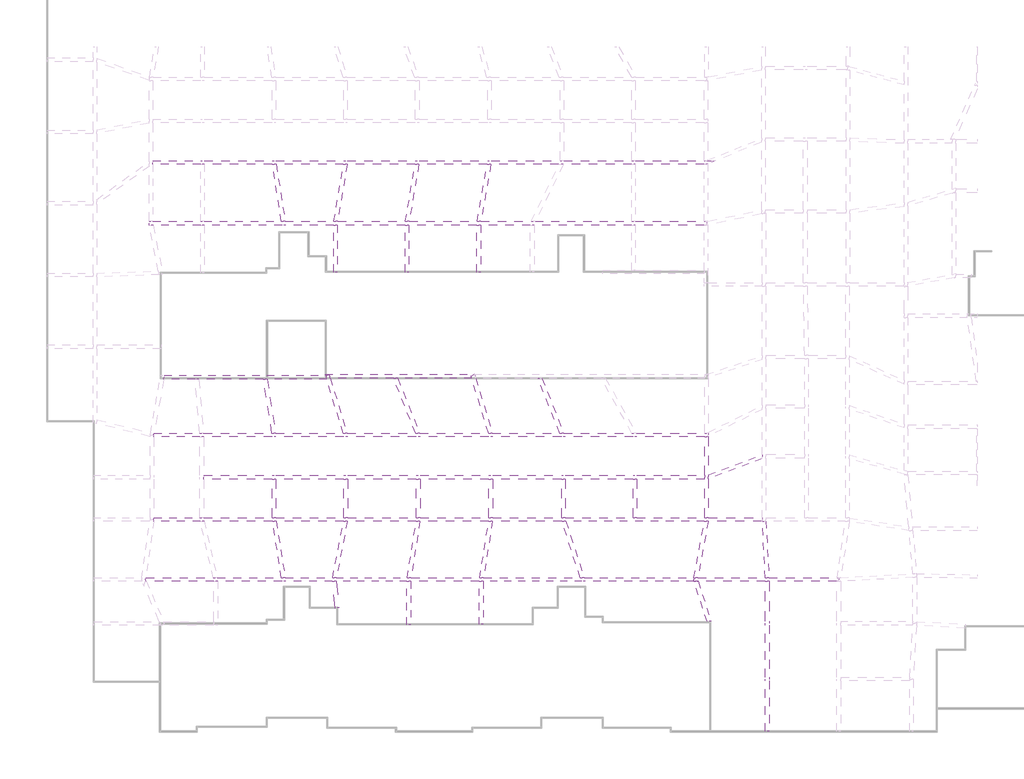
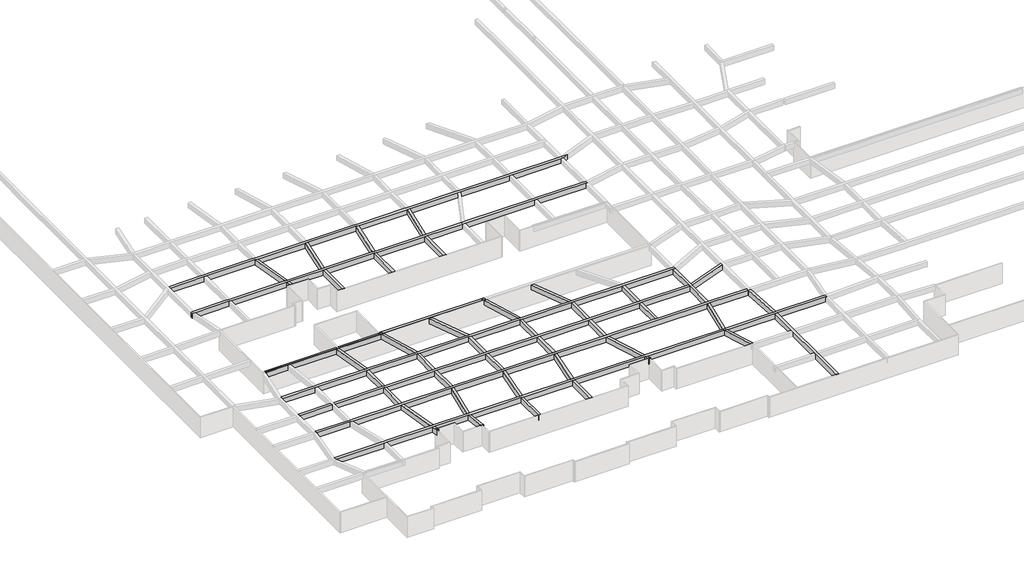
# One storey, part 11 of 45: 41 beams.
"""IFC4 building model written with IfcOpenShell, lengths in millimetres."""

from ifc_helpers import new_model, si_unit, frame, origin, place, context, project, spatial, polyline, outline, extrude, faceted_brep, element, save

model = new_model("IFC4")

# Units and contexts
model_context = context("Model", 3, world=origin())
ifc_project = project(units=[si_unit("LENGTHUNIT", "METRE", prefix="MILLI")], contexts=[model_context])

# Site, building, storey
site = spatial("IfcSite", under=ifc_project)
building = spatial("IfcBuilding", under=site)
storey = spatial("IfcBuildingStorey", under=building, Name="户型图", Elevation=0.0)

# Beams
placement = place(None, origin())
element("IfcBeam", 1, ObjectType="混凝土 - 矩形梁 : KL_beam", at=placement, inside=storey, context=model_context, shape_type="Brep", body=[
    faceted_brep([(-73789.7274974, -130269.3244435, 3300.0), (-73674.2267606, -130222.6591167, 3300.0), (-72799.6927561, -129869.3244435, 3300.0), (-73867.4796211, -129869.3244435, 3300.0), (-74074.2267606, -129869.3244435, 3300.0), (-81574.2267606, -129869.3244435, 3300.0), (-81974.2267606, -129869.3244435, 3300.0), (-89374.2267606, -129869.3244435, 3300.0), (-89774.2267606, -129869.3244435, 3300.0), (-97274.2267606, -129869.3244435, 3300.0), (-97674.2267606, -129869.3244435, 3300.0), (-105129.6078212, -129869.3244435, 3300.0), (-105529.6078212, -129869.3244435, 3300.0), (-112929.6078212, -129869.3244435, 3300.0), (-113329.6078212, -129869.3244435, 3300.0), (-120729.6078212, -129869.3244435, 3300.0), (-121129.6078212, -129869.3244435, 3300.0), (-128529.6078212, -129869.3244435, 3300.0), (-128929.6078212, -129869.3244435, 3300.0), (-134129.6078212, -129869.3244435, 3300.0), (-134129.6078212, -130269.3244435, 3300.0), (-128929.6078212, -130269.3244435, 3300.0), (-128529.6078212, -130269.3244435, 3300.0), (-121100.4239582, -130269.3244435, 3300.0), (-120695.4379079, -130269.3244435, 3300.0), (-113366.1859307, -130269.3244435, 3300.0), (-112960.5304704, -130269.3244435, 3300.0), (-105566.1859307, -130269.3244435, 3300.0), (-105160.5304704, -130269.3244435, 3300.0), (-97712.5774791, -130269.3244435, 3300.0), (-97306.4068344, -130269.3244435, 3300.0), (-89894.2936664, -130269.3244435, 3300.0), (-89449.2528902, -130269.3244435, 3300.0), (-81974.2267606, -130269.3244435, 3300.0), (-81574.2267606, -130269.3244435, 3300.0), (-74074.2267606, -130269.3244435, 3300.0), (-73789.7274974, -130269.3244435, 2500.0), (-134129.6078212, -130269.3244435, 2500.0), (-128929.6078212, -130269.3244435, 2500.0), (-128529.6078212, -130269.3244435, 2500.0), (-121100.4239582, -130269.3244435, 2500.0), (-120695.4379079, -130269.3244435, 2500.0), (-113366.1859307, -130269.3244435, 2500.0), (-112960.5304704, -130269.3244435, 2500.0), (-105566.1859307, -130269.3244435, 2500.0), (-105160.5304704, -130269.3244435, 2500.0), (-97712.5774791, -130269.3244435, 2500.0), (-97306.4068344, -130269.3244435, 2500.0), (-89894.2936664, -130269.3244435, 2500.0), (-89449.2528902, -130269.3244435, 2500.0), (-81974.2267606, -130269.3244435, 2500.0), (-81574.2267606, -130269.3244435, 2500.0), (-74074.2267606, -130269.3244435, 2500.0), (-72799.6927561, -129869.3244435, 2500.0), (-73674.2267606, -130222.6591167, 2500.0), (-134129.6078212, -129869.3244435, 2500.0), (-128929.6078212, -129869.3244435, 2500.0), (-128529.6078212, -129869.3244435, 2500.0), (-121129.6078212, -129869.3244435, 2500.0), (-120729.6078212, -129869.3244435, 2500.0), (-113329.6078212, -129869.3244435, 2500.0), (-112929.6078212, -129869.3244435, 2500.0), (-105529.6078212, -129869.3244435, 2500.0), (-105129.6078212, -129869.3244435, 2500.0), (-97674.2267606, -129869.3244435, 2500.0), (-97274.2267606, -129869.3244435, 2500.0), (-89774.2267606, -129869.3244435, 2500.0), (-89374.2267606, -129869.3244435, 2500.0), (-81974.2267606, -129869.3244435, 2500.0), (-81574.2267606, -129869.3244435, 2500.0), (-74074.2267606, -129869.3244435, 2500.0), (-73867.4796211, -129869.3244435, 2500.0)], [[[0, 1, 2, 3, 4, 5, 6, 7, 8, 9, 10, 11, 12, 13, 14, 15, 16, 17, 18, 19, 20, 21, 22, 23, 24, 25, 26, 27, 28, 29, 30, 31, 32, 33, 34, 35]], [[36, 0, 35, 34, 33, 32, 31, 30, 29, 28, 27, 26, 25, 24, 23, 22, 21, 20, 37, 38, 39, 40, 41, 42, 43, 44, 45, 46, 47, 48, 49, 50, 51, 52]], [[53, 54, 36, 52, 51, 50, 49, 48, 47, 46, 45, 44, 43, 42, 41, 40, 39, 38, 37, 55, 56, 57, 58, 59, 60, 61, 62, 63, 64, 65, 66, 67, 68, 69, 70, 71]], [[2, 53, 71, 70, 69, 68, 67, 66, 65, 64, 63, 62, 61, 60, 59, 58, 57, 56, 55, 19, 18, 17, 16, 15, 14, 13, 12, 11, 10, 9, 8, 7, 6, 5, 4, 3]], [[20, 19, 55, 37]], [[2, 1, 0, 36, 54, 53]]]),
])
element("IfcBeam", 2, ObjectType="混凝土 - 矩形梁 : KL_beam", at=placement, inside=storey, context=model_context, shape_type="Brep", body=[
    faceted_brep([(-73801.0394369, -136882.7394466, 3300.0), (-73841.6921627, -136482.7394466, 3300.0), (-74074.2267606, -136482.7394466, 3300.0), (-81574.2267606, -136482.7394466, 3300.0), (-81974.2267606, -136482.7394466, 3300.0), (-92479.7378735, -136482.7394466, 3300.0), (-92924.7786497, -136482.7394466, 3300.0), (-98401.9995417, -136482.7394466, 3300.0), (-98808.1701865, -136482.7394466, 3300.0), (-106209.0560389, -136482.7394466, 3300.0), (-106614.7114991, -136482.7394466, 3300.0), (-114009.0560389, -136482.7394466, 3300.0), (-114414.7114991, -136482.7394466, 3300.0), (-119711.3296502, -136482.7394466, 3300.0), (-120116.3157005, -136482.7394466, 3300.0), (-128529.6078212, -136482.7394466, 3300.0), (-128929.6078212, -136482.7394466, 3300.0), (-134129.6078212, -136482.7394466, 3300.0), (-134529.6078212, -136482.7394466, 3300.0), (-134529.6078212, -136882.7394466, 3300.0), (-134494.0876303, -136882.7394466, 3300.0), (-134086.4357741, -136882.7394466, 3300.0), (-128929.6078212, -136882.7394466, 3300.0), (-128529.6078212, -136882.7394466, 3300.0), (-120052.9619243, -136882.7394466, 3300.0), (-119647.975874, -136882.7394466, 3300.0), (-114445.6408237, -136882.7394466, 3300.0), (-114045.6408237, -136882.7394466, 3300.0), (-106645.6408237, -136882.7394466, 3300.0), (-106245.6408237, -136882.7394466, 3300.0), (-98840.399091, -136882.7394466, 3300.0), (-98440.399091, -136882.7394466, 3300.0), (-93000.0024046, -136882.7394466, 3300.0), (-92600.0024046, -136882.7394466, 3300.0), (-81974.2267606, -136882.7394466, 3300.0), (-81574.2267606, -136882.7394466, 3300.0), (-74074.2267606, -136882.7394466, 3300.0), (-73801.0394369, -136882.7394466, 2500.0), (-134529.6078212, -136882.7394466, 2500.0), (-134494.0876303, -136882.7394466, 2500.0), (-134086.4357741, -136882.7394466, 2500.0), (-128929.6078212, -136882.7394466, 2500.0), (-128529.6078212, -136882.7394466, 2500.0), (-120052.9619243, -136882.7394466, 2500.0), (-119647.975874, -136882.7394466, 2500.0), (-114445.6408237, -136882.7394466, 2500.0), (-114045.6408237, -136882.7394466, 2500.0), (-106645.6408237, -136882.7394466, 2500.0), (-106245.6408237, -136882.7394466, 2500.0), (-98840.399091, -136882.7394466, 2500.0), (-98440.399091, -136882.7394466, 2500.0), (-93000.0024046, -136882.7394466, 2500.0), (-92600.0024046, -136882.7394466, 2500.0), (-81974.2267606, -136882.7394466, 2500.0), (-81574.2267606, -136882.7394466, 2500.0), (-74074.2267606, -136882.7394466, 2500.0), (-73841.6921627, -136482.7394466, 2500.0), (-134529.6078212, -136482.7394466, 2500.0), (-134129.6078212, -136482.7394466, 2500.0), (-128929.6078212, -136482.7394466, 2500.0), (-128529.6078212, -136482.7394466, 2500.0), (-120116.3157005, -136482.7394466, 2500.0), (-119711.3296502, -136482.7394466, 2500.0), (-114414.7114991, -136482.7394466, 2500.0), (-114009.0560389, -136482.7394466, 2500.0), (-106614.7114991, -136482.7394466, 2500.0), (-106209.0560389, -136482.7394466, 2500.0), (-98808.1701865, -136482.7394466, 2500.0), (-98401.9995417, -136482.7394466, 2500.0), (-92924.7786497, -136482.7394466, 2500.0), (-92479.7378735, -136482.7394466, 2500.0), (-81974.2267606, -136482.7394466, 2500.0), (-81574.2267606, -136482.7394466, 2500.0), (-74074.2267606, -136482.7394466, 2500.0)], [[[0, 1, 2, 3, 4, 5, 6, 7, 8, 9, 10, 11, 12, 13, 14, 15, 16, 17, 18, 19, 20, 21, 22, 23, 24, 25, 26, 27, 28, 29, 30, 31, 32, 33, 34, 35, 36]], [[37, 0, 36, 35, 34, 33, 32, 31, 30, 29, 28, 27, 26, 25, 24, 23, 22, 21, 20, 19, 38, 39, 40, 41, 42, 43, 44, 45, 46, 47, 48, 49, 50, 51, 52, 53, 54, 55]], [[56, 37, 55, 54, 53, 52, 51, 50, 49, 48, 47, 46, 45, 44, 43, 42, 41, 40, 39, 38, 57, 58, 59, 60, 61, 62, 63, 64, 65, 66, 67, 68, 69, 70, 71, 72, 73]], [[1, 56, 73, 72, 71, 70, 69, 68, 67, 66, 65, 64, 63, 62, 61, 60, 59, 58, 57, 18, 17, 16, 15, 14, 13, 12, 11, 10, 9, 8, 7, 6, 5, 4, 3, 2]], [[19, 18, 57, 38]], [[1, 0, 37, 56]]]),
])
element("IfcBeam", 3, ObjectType="混凝土 - 矩形梁 : KL_beam", at=placement, inside=storey, context=model_context, shape_type="SweptSolid", body=[
    extrude(outline(polyline([(-105566.1859307, -130269.3244435), (-105160.5304704, -130269.3244435), (-106209.0560389, -136482.7394466), (-106614.7114991, -136482.7394466), (-105566.1859307, -130269.3244435)])), frame((0.0, 0.0, 2500.0), z_axis=(0.0, 0.0, 1.0), x_axis=(1.0, 0.0, 0.0)), (0.0, 0.0, 1.0), 800.0),
])
element("IfcBeam", 4, ObjectType="混凝土 - 矩形梁 : KL_beam", at=placement, inside=storey, context=model_context, shape_type="SweptSolid", body=[
    extrude(outline(polyline([(-113366.1859307, -130269.3244435), (-112960.5304704, -130269.3244435), (-114009.0560389, -136482.7394466), (-114414.7114991, -136482.7394466), (-113366.1859307, -130269.3244435)])), frame((0.0, 0.0, 2500.0), z_axis=(0.0, 0.0, 1.0), x_axis=(1.0, 0.0, 0.0)), (0.0, 0.0, 1.0), 800.0),
])
element("IfcBeam", 5, ObjectType="混凝土 - 矩形梁 : KL_beam", at=placement, inside=storey, context=model_context, shape_type="SweptSolid", body=[
    extrude(outline(polyline([(-97712.5774791, -130269.3244435), (-97306.4068344, -130269.3244435), (-98401.9995417, -136482.7394466), (-98808.1701865, -136482.7394466), (-97712.5774791, -130269.3244435)])), frame((0.0, 0.0, 2500.0), z_axis=(0.0, 0.0, 1.0), x_axis=(1.0, 0.0, 0.0)), (0.0, 0.0, 1.0), 800.0),
])
element("IfcBeam", 6, ObjectType="混凝土 - 矩形梁 : KL_beam", at=placement, inside=storey, context=model_context, shape_type="SweptSolid", body=[
    extrude(outline(polyline([(-98440.399091, -141990.9010637), (-98840.399091, -141990.9010637), (-98840.399091, -136882.7394466), (-98440.399091, -136882.7394466), (-98440.399091, -141990.9010637)])), frame((0.0, 0.0, 2500.0), z_axis=(0.0, 0.0, 1.0), x_axis=(1.0, 0.0, 0.0)), (0.0, 0.0, 1.0), 800.0),
])
element("IfcBeam", 7, ObjectType="混凝土 - 矩形梁 : KL_beam", at=placement, inside=storey, context=model_context, shape_type="Brep", body=[
    faceted_brep([(-75195.4874183, -175680.7215365, 3300.0), (-74862.8225004, -175680.7215365, 3300.0), (-74755.4433093, -175680.7215365, 3300.0), (-67421.4283331, -175680.7215365, 3300.0), (-67021.4283331, -175680.7215365, 3300.0), (-59629.7273676, -175680.7215365, 3300.0), (-59424.4901833, -175680.7215365, 3300.0), (-59434.9645519, -175280.7215365, 3300.0), (-59602.3197398, -175280.7215365, 3300.0), (-67031.6354197, -175280.7215365, 3300.0), (-67432.1843581, -175280.7215365, 3300.0), (-74788.6727332, -175280.7215365, 3300.0), (-75195.4874183, -175280.7215365, 3300.0), (-75195.4874183, -175283.8093857, 3300.0), (-59434.9645519, -175280.7215365, 2500.0), (-59602.3197398, -175280.7215365, 2500.0), (-67031.6354197, -175280.7215365, 2500.0), (-67432.1843581, -175280.7215365, 2500.0), (-74788.6727332, -175280.7215365, 2500.0), (-75195.4874183, -175280.7215365, 2500.0), (-59424.4901833, -175680.7215365, 2500.0), (-59629.7273676, -175680.7215365, 2500.0), (-67021.4283331, -175680.7215365, 2500.0), (-67421.4283331, -175680.7215365, 2500.0), (-74755.4433093, -175680.7215365, 2500.0), (-74862.8225004, -175680.7215365, 2500.0), (-75195.4874183, -175680.7215365, 2500.0), (-75195.4874183, -175283.8093857, 2500.0)], [[[0, 1, 2, 3, 4, 5, 6, 7, 8, 9, 10, 11, 12, 13]], [[12, 11, 10, 9, 8, 7, 14, 15, 16, 17, 18, 19]], [[19, 18, 17, 16, 15, 14, 20, 21, 22, 23, 24, 25, 26, 27]], [[6, 5, 4, 3, 2, 1, 0, 26, 25, 24, 23, 22, 21, 20]], [[6, 20, 14, 7]], [[0, 13, 12, 19, 27, 26]]]),
])
element("IfcBeam", 8, ObjectType="混凝土 - 矩形梁 : KL_beam", at=placement, inside=storey, context=model_context, shape_type="Brep", body=[
    faceted_brep([(-67352.9383994, -169149.8954633, 3300.0), (-67363.6944245, -169149.8954633, 3300.0), (-67753.4873378, -169149.8954633, 3300.0), (-67432.1843581, -175280.7215365, 3300.0), (-67031.6354197, -175280.7215365, 3300.0), (-67753.4873378, -169149.8954633, 2500.0), (-67432.1843581, -175280.7215365, 2500.0), (-67363.6944245, -169149.8954633, 2500.0), (-67352.9383994, -169149.8954633, 2500.0), (-67031.6354197, -175280.7215365, 2500.0)], [[[0, 1, 2, 3, 4]], [[2, 5, 6, 3]], [[5, 7, 8, 9, 6]], [[8, 0, 4, 9]], [[5, 2, 1, 0, 8, 7]], [[4, 3, 6, 9]]]),
    faceted_brep([(-67763.6944245, -168955.1326476, 3300.0), (-67763.6944245, -168955.1326476, 2500.0), (-67763.6944245, -168749.8954633, 2500.0), (-67763.6944245, -168748.040132, 2500.0), (-67763.6944245, -168748.040132, 3300.0), (-67763.6944245, -168749.8954633, 3300.0), (-67774.5476833, -168748.040132, 2500.0), (-67774.5476833, -168748.040132, 3300.0)], [[[0, 1, 2, 3, 4, 5]], [[6, 7, 4, 3]], [[7, 0, 5, 4]], [[0, 7, 6, 1]], [[1, 6, 3, 2]]]),
])
element("IfcBeam", 9, ObjectType="混凝土 - 矩形梁 : KL_beam", at=placement, inside=storey, context=model_context, shape_type="Brep", body=[
    faceted_brep([(-67021.4283331, -192027.8669315, 3300.0), (-67421.4283331, -192027.8669315, 3300.0), (-67421.4283331, -192027.8669315, 2500.0), (-67021.4283331, -192027.8669315, 2500.0), (-67021.4283331, -186528.0123265, 3300.0), (-67021.4283331, -186128.0123265, 3300.0), (-67021.4283331, -180443.730522, 3300.0), (-67021.4283331, -180043.730522, 3300.0), (-67021.4283331, -175680.7215365, 3300.0), (-67421.4283331, -175680.7215365, 3300.0), (-67421.4283331, -180043.730522, 3300.0), (-67421.4283331, -180443.730522, 3300.0), (-67421.4283331, -186128.0123265, 3300.0), (-67421.4283331, -186528.0123265, 3300.0), (-67421.4283331, -175680.7215365, 2500.0), (-67421.4283331, -180043.730522, 2500.0), (-67421.4283331, -180443.730522, 2500.0), (-67421.4283331, -186128.0123265, 2500.0), (-67421.4283331, -186528.0123265, 2500.0), (-67021.4283331, -175680.7215365, 2500.0), (-67021.4283331, -180043.730522, 2500.0), (-67021.4283331, -180443.730522, 2500.0), (-67021.4283331, -186128.0123265, 2500.0), (-67021.4283331, -186528.0123265, 2500.0)], [[[0, 1, 2, 3]], [[1, 0, 4, 5, 6, 7, 8, 9, 10, 11, 12, 13]], [[2, 1, 13, 12, 11, 10, 9, 14, 15, 16, 17, 18]], [[3, 2, 18, 17, 16, 15, 14, 19, 20, 21, 22, 23]], [[0, 3, 23, 22, 21, 20, 19, 8, 7, 6, 5, 4]], [[9, 8, 19, 14]]]),
])
element("IfcBeam", 10, ObjectType="混凝土 - 矩形梁 : KL_beam", at=placement, inside=storey, context=model_context, shape_type="SweptSolid", body=[
    extrude(outline(polyline([(-119527.5247722, -137643.237773), (-119922.6001085, -137705.8115591), (-120052.9619243, -136882.7394466), (-119647.975874, -136882.7394466), (-119527.5247722, -137643.237773)])), frame((0.0, 0.0, 2500.0), z_axis=(0.0, 0.0, 1.0), x_axis=(1.0, 0.0, 0.0)), (0.0, 0.0, 1.0), 800.0),
    extrude(outline(polyline([(-121100.4239582, -130269.3244435), (-120695.4379079, -130269.3244435), (-119711.3296502, -136482.7394466), (-120116.3157005, -136482.7394466), (-121100.4239582, -130269.3244435)])), frame((0.0, 0.0, 2500.0), z_axis=(0.0, 0.0, 1.0), x_axis=(1.0, 0.0, 0.0)), (0.0, 0.0, 1.0), 800.0),
])
element("IfcBeam", 11, ObjectType="混凝土 - 矩形梁 : KL_beam", at=placement, inside=storey, context=model_context, shape_type="Brep", body=[
    faceted_brep([(-134906.6317316, -175283.8093857, 3300.0), (-134930.932576, -175456.7188778, 3300.0), (-134834.5383744, -175683.8093857, 3300.0), (-127468.1198938, -175683.8093857, 3300.0), (-127068.1198938, -175683.8093857, 3300.0), (-120053.8149285, -175683.8093857, 3300.0), (-119648.8288782, -175683.8093857, 3300.0), (-114567.3022088, -175683.8093857, 3300.0), (-114164.7670122, -175683.8093857, 3300.0), (-106453.3866692, -175683.8093857, 3300.0), (-106053.3866692, -175683.8093857, 3300.0), (-98553.3271021, -175683.8093857, 3300.0), (-98153.3271021, -175683.8093857, 3300.0), (-87439.8712918, -175683.8093857, 3300.0), (-87019.2864021, -175683.8093857, 3300.0), (-75175.0248959, -175683.8093857, 3300.0), (-74863.3949086, -175683.8093857, 3300.0), (-74862.8225004, -175680.7215365, 3300.0), (-75195.4874183, -175680.7215365, 3300.0), (-75195.4874183, -175283.8093857, 3300.0), (-87149.2542806, -175283.8093857, 3300.0), (-87569.8391703, -175283.8093857, 3300.0), (-98119.1571889, -175283.8093857, 3300.0), (-98524.1432392, -175283.8093857, 3300.0), (-106019.1571889, -175283.8093857, 3300.0), (-106424.1432392, -175283.8093857, 3300.0), (-114145.9683939, -175283.8093857, 3300.0), (-114553.4550719, -175283.8093857, 3300.0), (-119712.1826543, -175283.8093857, 3300.0), (-120117.1687046, -175283.8093857, 3300.0), (-127122.7494049, -175283.8093857, 3300.0), (-127533.271048, -175283.8093857, 3300.0), (-134834.5383744, -175683.8093857, 2500.0), (-127468.1198938, -175683.8093857, 2500.0), (-127068.1198938, -175683.8093857, 2500.0), (-120053.8149285, -175683.8093857, 2500.0), (-119648.8288782, -175683.8093857, 2500.0), (-114567.3022088, -175683.8093857, 2500.0), (-114164.7670122, -175683.8093857, 2500.0), (-106453.3866692, -175683.8093857, 2500.0), (-106053.3866692, -175683.8093857, 2500.0), (-98553.3271021, -175683.8093857, 2500.0), (-98153.3271021, -175683.8093857, 2500.0), (-87439.8712918, -175683.8093857, 2500.0), (-87019.2864021, -175683.8093857, 2500.0), (-75175.0248959, -175683.8093857, 2500.0), (-74863.3949086, -175683.8093857, 2500.0), (-134930.932576, -175456.7188778, 2500.0), (-134906.6317316, -175283.8093857, 2500.0), (-127533.271048, -175283.8093857, 2500.0), (-127122.7494049, -175283.8093857, 2500.0), (-120117.1687046, -175283.8093857, 2500.0), (-119712.1826543, -175283.8093857, 2500.0), (-114553.4550719, -175283.8093857, 2500.0), (-114145.9683939, -175283.8093857, 2500.0), (-106424.1432392, -175283.8093857, 2500.0), (-106019.1571889, -175283.8093857, 2500.0), (-98524.1432392, -175283.8093857, 2500.0), (-98119.1571889, -175283.8093857, 2500.0), (-87569.8391703, -175283.8093857, 2500.0), (-87149.2542806, -175283.8093857, 2500.0), (-75195.4874183, -175283.8093857, 2500.0), (-75195.4874183, -175680.7215365, 2500.0), (-74862.8225004, -175680.7215365, 2500.0)], [[[0, 1, 2, 3, 4, 5, 6, 7, 8, 9, 10, 11, 12, 13, 14, 15, 16, 17, 18, 19, 20, 21, 22, 23, 24, 25, 26, 27, 28, 29, 30, 31]], [[2, 32, 33, 34, 35, 36, 37, 38, 39, 40, 41, 42, 43, 44, 45, 46, 16, 15, 14, 13, 12, 11, 10, 9, 8, 7, 6, 5, 4, 3]], [[47, 48, 49, 50, 51, 52, 53, 54, 55, 56, 57, 58, 59, 60, 61, 62, 63, 46, 45, 44, 43, 42, 41, 40, 39, 38, 37, 36, 35, 34, 33, 32]], [[48, 0, 31, 30, 29, 28, 27, 26, 25, 24, 23, 22, 21, 20, 19, 61, 60, 59, 58, 57, 56, 55, 54, 53, 52, 51, 50, 49]], [[0, 48, 47, 1]], [[2, 1, 47, 32]], [[62, 18, 17, 63]], [[18, 62, 61, 19]], [[16, 46, 63, 17]]]),
])
element("IfcBeam", 12, ObjectType="混凝土 - 矩形梁 : KL_beam", at=placement, inside=storey, context=model_context, shape_type="Brep", body=[
    faceted_brep([(-67763.6944245, -169148.040132, 3300.0), (-67763.6944245, -168955.1326476, 3300.0), (-67774.5476833, -168748.040132, 3300.0), (-73618.1629467, -168748.040132, 3300.0), (-74018.1629467, -168748.040132, 3300.0), (-81418.1629467, -168748.040132, 3300.0), (-81818.1629467, -168748.040132, 3300.0), (-89218.1629467, -168748.040132, 3300.0), (-89618.1629467, -168748.040132, 3300.0), (-97118.1629467, -168748.040132, 3300.0), (-97518.1629467, -168748.040132, 3300.0), (-105018.1629467, -168748.040132, 3300.0), (-105418.1629467, -168748.040132, 3300.0), (-112918.1629467, -168748.040132, 3300.0), (-113318.1629467, -168748.040132, 3300.0), (-120718.1629467, -168748.040132, 3300.0), (-121118.1629467, -168748.040132, 3300.0), (-128597.7870634, -168748.040132, 3300.0), (-128997.7870634, -168748.040132, 3300.0), (-134018.1629467, -168748.040132, 3300.0), (-134018.1629467, -168962.0254944, 3300.0), (-134044.3055992, -169148.040132, 3300.0), (-128949.8249968, -169148.040132, 3300.0), (-128539.3033537, -169148.040132, 3300.0), (-121088.9790838, -169148.040132, 3300.0), (-120683.9930335, -169148.040132, 3300.0), (-113360.7823476, -169148.040132, 3300.0), (-112953.2956696, -169148.040132, 3300.0), (-105452.33286, -169148.040132, 3300.0), (-105047.3468096, -169148.040132, 3300.0), (-97552.33286, -169148.040132, 3300.0), (-97147.3468096, -169148.040132, 3300.0), (-89563.4714523, -169148.040132, 3300.0), (-89142.8865626, -169148.040132, 3300.0), (-74058.6451728, -169148.040132, 3300.0), (-73651.8304878, -169148.040132, 3300.0), (-67763.6944245, -169148.040132, 2500.0), (-134044.3055992, -169148.040132, 2500.0), (-128949.8249968, -169148.040132, 2500.0), (-128539.3033537, -169148.040132, 2500.0), (-121088.9790838, -169148.040132, 2500.0), (-120683.9930335, -169148.040132, 2500.0), (-113360.7823476, -169148.040132, 2500.0), (-112953.2956696, -169148.040132, 2500.0), (-105452.33286, -169148.040132, 2500.0), (-105047.3468096, -169148.040132, 2500.0), (-97552.33286, -169148.040132, 2500.0), (-97147.3468096, -169148.040132, 2500.0), (-89563.4714523, -169148.040132, 2500.0), (-89142.8865626, -169148.040132, 2500.0), (-74058.6451728, -169148.040132, 2500.0), (-73651.8304878, -169148.040132, 2500.0), (-67763.6944245, -168955.1326476, 2500.0), (-134018.1629467, -168962.0254944, 2500.0), (-134018.1629467, -168748.040132, 2500.0), (-128997.7870634, -168748.040132, 2500.0), (-128597.7870634, -168748.040132, 2500.0), (-121118.1629467, -168748.040132, 2500.0), (-120718.1629467, -168748.040132, 2500.0), (-113318.1629467, -168748.040132, 2500.0), (-112918.1629467, -168748.040132, 2500.0), (-105418.1629467, -168748.040132, 2500.0), (-105018.1629467, -168748.040132, 2500.0), (-97518.1629467, -168748.040132, 2500.0), (-97118.1629467, -168748.040132, 2500.0), (-89618.1629467, -168748.040132, 2500.0), (-89218.1629467, -168748.040132, 2500.0), (-81818.1629467, -168748.040132, 2500.0), (-81418.1629467, -168748.040132, 2500.0), (-74018.1629467, -168748.040132, 2500.0), (-73618.1629467, -168748.040132, 2500.0), (-67774.5476833, -168748.040132, 2500.0)], [[[0, 1, 2, 3, 4, 5, 6, 7, 8, 9, 10, 11, 12, 13, 14, 15, 16, 17, 18, 19, 20, 21, 22, 23, 24, 25, 26, 27, 28, 29, 30, 31, 32, 33, 34, 35]], [[36, 0, 35, 34, 33, 32, 31, 30, 29, 28, 27, 26, 25, 24, 23, 22, 21, 37, 38, 39, 40, 41, 42, 43, 44, 45, 46, 47, 48, 49, 50, 51]], [[52, 36, 51, 50, 49, 48, 47, 46, 45, 44, 43, 42, 41, 40, 39, 38, 37, 53, 54, 55, 56, 57, 58, 59, 60, 61, 62, 63, 64, 65, 66, 67, 68, 69, 70, 71]], [[2, 71, 70, 69, 68, 67, 66, 65, 64, 63, 62, 61, 60, 59, 58, 57, 56, 55, 54, 19, 18, 17, 16, 15, 14, 13, 12, 11, 10, 9, 8, 7, 6, 5, 4, 3]], [[0, 36, 52, 1]], [[2, 1, 52, 71]], [[20, 19, 54, 53]], [[21, 20, 53, 37]]]),
])
element("IfcBeam", 13, ObjectType="混凝土 - 矩形梁 : KL_beam", at=placement, inside=storey, context=model_context, shape_type="Brep", body=[
    faceted_brep([(-134018.1629467, -164148.040132, 3300.0), (-134018.1629467, -164548.040132, 3300.0), (-128997.7870634, -164548.040132, 3300.0), (-128997.7870634, -164148.040132, 3300.0), (-134018.1629467, -164548.040132, 2500.0), (-128997.7870634, -164548.040132, 2500.0), (-134018.1629467, -164148.040132, 2500.0), (-128997.7870634, -164148.040132, 2500.0)], [[[0, 1, 2, 3]], [[1, 4, 5, 2]], [[4, 6, 7, 5]], [[6, 0, 3, 7]], [[1, 0, 6, 4]], [[3, 2, 5, 7]]]),
    faceted_brep([(-128597.7870634, -164548.040132, 3300.0), (-128597.7870634, -164148.040132, 3300.0), (-128597.7870634, -164148.040132, 2500.0), (-128597.7870634, -164548.040132, 2500.0), (-121118.1629467, -164548.040132, 3300.0), (-120718.1629467, -164548.040132, 3300.0), (-113318.1629467, -164548.040132, 3300.0), (-112918.1629467, -164548.040132, 3300.0), (-105418.1629467, -164548.040132, 3300.0), (-105018.1629467, -164548.040132, 3300.0), (-97518.1629467, -164548.040132, 3300.0), (-97118.1629467, -164548.040132, 3300.0), (-89618.1629467, -164548.040132, 3300.0), (-89218.1629467, -164548.040132, 3300.0), (-81818.1629467, -164548.040132, 3300.0), (-81418.1629467, -164548.040132, 3300.0), (-74018.1629467, -164548.040132, 3300.0), (-74018.1629467, -164148.040132, 3300.0), (-81418.1629467, -164148.040132, 3300.0), (-81818.1629467, -164148.040132, 3300.0), (-89218.1629467, -164148.040132, 3300.0), (-89618.1629467, -164148.040132, 3300.0), (-97118.1629467, -164148.040132, 3300.0), (-97518.1629467, -164148.040132, 3300.0), (-105018.1629467, -164148.040132, 3300.0), (-105418.1629467, -164148.040132, 3300.0), (-112918.1629467, -164148.040132, 3300.0), (-113318.1629467, -164148.040132, 3300.0), (-120718.1629467, -164148.040132, 3300.0), (-121118.1629467, -164148.040132, 3300.0), (-121118.1629467, -164548.040132, 2500.0), (-120718.1629467, -164548.040132, 2500.0), (-113318.1629467, -164548.040132, 2500.0), (-112918.1629467, -164548.040132, 2500.0), (-105418.1629467, -164548.040132, 2500.0), (-105018.1629467, -164548.040132, 2500.0), (-97518.1629467, -164548.040132, 2500.0), (-97118.1629467, -164548.040132, 2500.0), (-89618.1629467, -164548.040132, 2500.0), (-89218.1629467, -164548.040132, 2500.0), (-81818.1629467, -164548.040132, 2500.0), (-81418.1629467, -164548.040132, 2500.0), (-74018.1629467, -164548.040132, 2500.0), (-121118.1629467, -164148.040132, 2500.0), (-120718.1629467, -164148.040132, 2500.0), (-113318.1629467, -164148.040132, 2500.0), (-112918.1629467, -164148.040132, 2500.0), (-105418.1629467, -164148.040132, 2500.0), (-105018.1629467, -164148.040132, 2500.0), (-97518.1629467, -164148.040132, 2500.0), (-97118.1629467, -164148.040132, 2500.0), (-89618.1629467, -164148.040132, 2500.0), (-89218.1629467, -164148.040132, 2500.0), (-81818.1629467, -164148.040132, 2500.0), (-81418.1629467, -164148.040132, 2500.0), (-74018.1629467, -164148.040132, 2500.0)], [[[0, 1, 2, 3]], [[1, 0, 4, 5, 6, 7, 8, 9, 10, 11, 12, 13, 14, 15, 16, 17, 18, 19, 20, 21, 22, 23, 24, 25, 26, 27, 28, 29]], [[0, 3, 30, 31, 32, 33, 34, 35, 36, 37, 38, 39, 40, 41, 42, 16, 15, 14, 13, 12, 11, 10, 9, 8, 7, 6, 5, 4]], [[3, 2, 43, 44, 45, 46, 47, 48, 49, 50, 51, 52, 53, 54, 55, 42, 41, 40, 39, 38, 37, 36, 35, 34, 33, 32, 31, 30]], [[2, 1, 29, 28, 27, 26, 25, 24, 23, 22, 21, 20, 19, 18, 17, 55, 54, 53, 52, 51, 50, 49, 48, 47, 46, 45, 44, 43]], [[17, 16, 42, 55]]]),
])
element("IfcBeam", 14, ObjectType="混凝土 - 矩形梁 : KL_beam", at=placement, inside=storey, context=model_context, shape_type="Brep", body=[
    faceted_brep([(-134018.1629467, -159765.5378647, 3300.0), (-134018.1629467, -159948.040132, 3300.0), (-128997.7870634, -159948.040132, 3300.0), (-128597.7870634, -159948.040132, 3300.0), (-121118.1629467, -159948.040132, 3300.0), (-120718.1629467, -159948.040132, 3300.0), (-113318.1629467, -159948.040132, 3300.0), (-112918.1629467, -159948.040132, 3300.0), (-105418.1629467, -159948.040132, 3300.0), (-105018.1629467, -159948.040132, 3300.0), (-97518.1629467, -159948.040132, 3300.0), (-97118.1629467, -159948.040132, 3300.0), (-89618.1629467, -159948.040132, 3300.0), (-89218.1629467, -159948.040132, 3300.0), (-81818.1629467, -159948.040132, 3300.0), (-81418.1629467, -159948.040132, 3300.0), (-74018.1629467, -159948.040132, 3300.0), (-73618.1629467, -159948.040132, 3300.0), (-73618.1629467, -159872.1626835, 3300.0), (-73618.1629467, -159548.040132, 3300.0), (-74018.1629467, -159548.040132, 3300.0), (-81500.4571592, -159548.040132, 3300.0), (-81957.9933056, -159548.040132, 3300.0), (-89382.3344157, -159548.040132, 3300.0), (-89812.6518859, -159548.040132, 3300.0), (-97143.220681, -159548.040132, 3300.0), (-97561.4973835, -159548.040132, 3300.0), (-105082.3344157, -159548.040132, 3300.0), (-105512.6518859, -159548.040132, 3300.0), (-112970.1707317, -159548.040132, 3300.0), (-113388.4474343, -159548.040132, 3300.0), (-120747.3468096, -159548.040132, 3300.0), (-121152.33286, -159548.040132, 3300.0), (-128611.8494798, -159548.040132, 3300.0), (-129013.3774148, -159548.040132, 3300.0), (-133979.8122282, -159548.040132, 3300.0), (-133988.5990803, -159597.8728462, 3300.0), (-134018.1629467, -159948.040132, 2500.0), (-128997.7870634, -159948.040132, 2500.0), (-128597.7870634, -159948.040132, 2500.0), (-121118.1629467, -159948.040132, 2500.0), (-120718.1629467, -159948.040132, 2500.0), (-113318.1629467, -159948.040132, 2500.0), (-112918.1629467, -159948.040132, 2500.0), (-105418.1629467, -159948.040132, 2500.0), (-105018.1629467, -159948.040132, 2500.0), (-97518.1629467, -159948.040132, 2500.0), (-97118.1629467, -159948.040132, 2500.0), (-89618.1629467, -159948.040132, 2500.0), (-89218.1629467, -159948.040132, 2500.0), (-81818.1629467, -159948.040132, 2500.0), (-81418.1629467, -159948.040132, 2500.0), (-74018.1629467, -159948.040132, 2500.0), (-73618.1629467, -159948.040132, 2500.0), (-134018.1629467, -159765.5378647, 2500.0), (-133988.5990803, -159597.8728462, 2500.0), (-133979.8122282, -159548.040132, 2500.0), (-129013.3774148, -159548.040132, 2500.0), (-128611.8494798, -159548.040132, 2500.0), (-121152.33286, -159548.040132, 2500.0), (-120747.3468096, -159548.040132, 2500.0), (-113388.4474343, -159548.040132, 2500.0), (-112970.1707317, -159548.040132, 2500.0), (-105512.6518859, -159548.040132, 2500.0), (-105082.3344157, -159548.040132, 2500.0), (-97561.4973835, -159548.040132, 2500.0), (-97143.220681, -159548.040132, 2500.0), (-89812.6518859, -159548.040132, 2500.0), (-89382.3344157, -159548.040132, 2500.0), (-81957.9933056, -159548.040132, 2500.0), (-81500.4571592, -159548.040132, 2500.0), (-74018.1629467, -159548.040132, 2500.0), (-73618.1629467, -159548.040132, 2500.0), (-73618.1629467, -159872.1626835, 2500.0)], [[[0, 1, 2, 3, 4, 5, 6, 7, 8, 9, 10, 11, 12, 13, 14, 15, 16, 17, 18, 19, 20, 21, 22, 23, 24, 25, 26, 27, 28, 29, 30, 31, 32, 33, 34, 35, 36]], [[1, 37, 38, 39, 40, 41, 42, 43, 44, 45, 46, 47, 48, 49, 50, 51, 52, 53, 17, 16, 15, 14, 13, 12, 11, 10, 9, 8, 7, 6, 5, 4, 3, 2]], [[37, 54, 55, 56, 57, 58, 59, 60, 61, 62, 63, 64, 65, 66, 67, 68, 69, 70, 71, 72, 73, 53, 52, 51, 50, 49, 48, 47, 46, 45, 44, 43, 42, 41, 40, 39, 38]], [[56, 35, 34, 33, 32, 31, 30, 29, 28, 27, 26, 25, 24, 23, 22, 21, 20, 19, 72, 71, 70, 69, 68, 67, 66, 65, 64, 63, 62, 61, 60, 59, 58, 57]], [[35, 56, 55, 54, 0, 36]], [[1, 0, 54, 37]], [[19, 18, 17, 53, 73, 72]]]),
])
element("IfcBeam", 15, ObjectType="混凝土 - 矩形梁 : KL_beam", at=placement, inside=storey, context=model_context, shape_type="SweptSolid", body=[
    extrude(outline(polyline([(-121118.1629467, -159948.040132), (-120718.1629467, -159948.040132), (-120718.1629467, -164148.040132), (-121118.1629467, -164148.040132), (-121118.1629467, -159948.040132)])), frame((0.0, 0.0, 2500.0), z_axis=(0.0, 0.0, 1.0), x_axis=(1.0, 0.0, 0.0)), (0.0, 0.0, 1.0), 800.0),
    extrude(outline(polyline([(-120718.1629467, -168748.040132), (-121118.1629467, -168748.040132), (-121118.1629467, -164548.040132), (-120718.1629467, -164548.040132), (-120718.1629467, -168748.040132)])), frame((0.0, 0.0, 2500.0), z_axis=(0.0, 0.0, 1.0), x_axis=(1.0, 0.0, 0.0)), (0.0, 0.0, 1.0), 800.0),
])
element("IfcBeam", 16, ObjectType="混凝土 - 矩形梁 : KL_beam", at=placement, inside=storey, context=model_context, shape_type="SweptSolid", body=[
    extrude(outline(polyline([(-113318.1629467, -159948.040132), (-112918.1629467, -159948.040132), (-112918.1629467, -164148.040132), (-113318.1629467, -164148.040132), (-113318.1629467, -159948.040132)])), frame((0.0, 0.0, 2500.0), z_axis=(0.0, 0.0, 1.0), x_axis=(1.0, 0.0, 0.0)), (0.0, 0.0, 1.0), 800.0),
    extrude(outline(polyline([(-112918.1629467, -168748.040132), (-113318.1629467, -168748.040132), (-113318.1629467, -164548.040132), (-112918.1629467, -164548.040132), (-112918.1629467, -168748.040132)])), frame((0.0, 0.0, 2500.0), z_axis=(0.0, 0.0, 1.0), x_axis=(1.0, 0.0, 0.0)), (0.0, 0.0, 1.0), 800.0),
])
element("IfcBeam", 17, ObjectType="混凝土 - 矩形梁 : KL_beam", at=placement, inside=storey, context=model_context, shape_type="SweptSolid", body=[
    extrude(outline(polyline([(-105418.1629467, -159948.040132), (-105018.1629467, -159948.040132), (-105018.1629467, -164148.040132), (-105418.1629467, -164148.040132), (-105418.1629467, -159948.040132)])), frame((0.0, 0.0, 2500.0), z_axis=(0.0, 0.0, 1.0), x_axis=(1.0, 0.0, 0.0)), (0.0, 0.0, 1.0), 800.0),
    extrude(outline(polyline([(-105018.1629467, -168748.040132), (-105418.1629467, -168748.040132), (-105418.1629467, -164548.040132), (-105018.1629467, -164548.040132), (-105018.1629467, -168748.040132)])), frame((0.0, 0.0, 2500.0), z_axis=(0.0, 0.0, 1.0), x_axis=(1.0, 0.0, 0.0)), (0.0, 0.0, 1.0), 800.0),
])
element("IfcBeam", 18, ObjectType="混凝土 - 矩形梁 : KL_beam", at=placement, inside=storey, context=model_context, shape_type="SweptSolid", body=[
    extrude(outline(polyline([(-97518.1629467, -159948.040132), (-97118.1629467, -159948.040132), (-97118.1629467, -164148.040132), (-97518.1629467, -164148.040132), (-97518.1629467, -159948.040132)])), frame((0.0, 0.0, 2500.0), z_axis=(0.0, 0.0, 1.0), x_axis=(1.0, 0.0, 0.0)), (0.0, 0.0, 1.0), 800.0),
    extrude(outline(polyline([(-97118.1629467, -168748.040132), (-97518.1629467, -168748.040132), (-97518.1629467, -164548.040132), (-97118.1629467, -164548.040132), (-97118.1629467, -168748.040132)])), frame((0.0, 0.0, 2500.0), z_axis=(0.0, 0.0, 1.0), x_axis=(1.0, 0.0, 0.0)), (0.0, 0.0, 1.0), 800.0),
])
element("IfcBeam", 19, ObjectType="混凝土 - 矩形梁 : KL_beam", at=placement, inside=storey, context=model_context, shape_type="SweptSolid", body=[
    extrude(outline(polyline([(-89618.1629467, -159948.040132), (-89218.1629467, -159948.040132), (-89218.1629467, -164148.040132), (-89618.1629467, -164148.040132), (-89618.1629467, -159948.040132)])), frame((0.0, 0.0, 2500.0), z_axis=(0.0, 0.0, 1.0), x_axis=(1.0, 0.0, 0.0)), (0.0, 0.0, 1.0), 800.0),
    extrude(outline(polyline([(-89218.1629467, -168748.040132), (-89618.1629467, -168748.040132), (-89618.1629467, -164548.040132), (-89218.1629467, -164548.040132), (-89218.1629467, -168748.040132)])), frame((0.0, 0.0, 2500.0), z_axis=(0.0, 0.0, 1.0), x_axis=(1.0, 0.0, 0.0)), (0.0, 0.0, 1.0), 800.0),
])
element("IfcBeam", 20, ObjectType="混凝土 - 矩形梁 : KL_beam", at=placement, inside=storey, context=model_context, shape_type="SweptSolid", body=[
    extrude(outline(polyline([(-81818.1629467, -159948.040132), (-81418.1629467, -159948.040132), (-81418.1629467, -164148.040132), (-81818.1629467, -164148.040132), (-81818.1629467, -159948.040132)])), frame((0.0, 0.0, 2500.0), z_axis=(0.0, 0.0, 1.0), x_axis=(1.0, 0.0, 0.0)), (0.0, 0.0, 1.0), 800.0),
    extrude(outline(polyline([(-81418.1629467, -168748.040132), (-81818.1629467, -168748.040132), (-81818.1629467, -164548.040132), (-81418.1629467, -164548.040132), (-81418.1629467, -168748.040132)])), frame((0.0, 0.0, 2500.0), z_axis=(0.0, 0.0, 1.0), x_axis=(1.0, 0.0, 0.0)), (0.0, 0.0, 1.0), 800.0),
])
element("IfcBeam", 21, ObjectType="混凝土 - 矩形梁 : KL_beam", at=placement, inside=storey, context=model_context, shape_type="Brep", body=[
    faceted_brep([(-73618.1629467, -159948.040132, 3300.0), (-74018.1629467, -159948.040132, 3300.0), (-74018.1629467, -164148.040132, 3300.0), (-74018.1629467, -164548.040132, 3300.0), (-74018.1629467, -168748.040132, 3300.0), (-73618.1629467, -168748.040132, 3300.0), (-73618.1629467, -164487.6259726, 3300.0), (-73618.1629467, -164061.4781152, 3300.0), (-74018.1629467, -159948.040132, 2500.0), (-74018.1629467, -164148.040132, 2500.0), (-74018.1629467, -164548.040132, 2500.0), (-74018.1629467, -168748.040132, 2500.0), (-73618.1629467, -159948.040132, 2500.0), (-73618.1629467, -164061.4781152, 2500.0), (-73618.1629467, -164487.6259726, 2500.0), (-73618.1629467, -168748.040132, 2500.0)], [[[0, 1, 2, 3, 4, 5, 6, 7]], [[1, 8, 9, 10, 11, 4, 3, 2]], [[8, 12, 13, 14, 15, 11, 10, 9]], [[12, 0, 7, 6, 5, 15, 14, 13]], [[1, 0, 12, 8]], [[5, 4, 11, 15]]]),
])
element("IfcBeam", 22, ObjectType="混凝土 - 矩形梁 : KL_beam", at=placement, inside=storey, context=model_context, shape_type="SweptSolid", body=[
    extrude(outline(polyline([(-74788.6727332, -175280.7215365), (-75195.4874183, -175280.7215365), (-74058.6451728, -169148.040132), (-73651.8304878, -169148.040132), (-74788.6727332, -175280.7215365)])), frame((0.0, 0.0, 2500.0), z_axis=(0.0, 0.0, 1.0), x_axis=(1.0, 0.0, 0.0)), (0.0, 0.0, 1.0), 800.0),
])
element("IfcBeam", 23, ObjectType="混凝土 - 矩形梁 : KL_beam", at=placement, inside=storey, context=model_context, shape_type="SweptSolid", body=[
    extrude(outline(polyline([(-86817.6190874, -176304.4775603), (-87198.0416939, -176428.084358), (-87439.8712918, -175683.8093857), (-87019.2864021, -175683.8093857), (-86817.6190874, -176304.4775603)])), frame((0.0, 0.0, 2500.0), z_axis=(0.0, 0.0, 1.0), x_axis=(1.0, 0.0, 0.0)), (0.0, 0.0, 1.0), 800.0),
    extrude(outline(polyline([(-89563.4714523, -169148.040132), (-89142.8865626, -169148.040132), (-87149.2542806, -175283.8093857), (-87569.8391703, -175283.8093857), (-89563.4714523, -169148.040132)])), frame((0.0, 0.0, 2500.0), z_axis=(0.0, 0.0, 1.0), x_axis=(1.0, 0.0, 0.0)), (0.0, 0.0, 1.0), 800.0),
])
element("IfcBeam", 24, ObjectType="混凝土 - 矩形梁 : KL_beam", at=placement, inside=storey, context=model_context, shape_type="SweptSolid", body=[
    extrude(outline(polyline([(-98119.1571889, -175283.8093857), (-98524.1432392, -175283.8093857), (-97552.33286, -169148.040132), (-97147.3468096, -169148.040132), (-98119.1571889, -175283.8093857)])), frame((0.0, 0.0, 2500.0), z_axis=(0.0, 0.0, 1.0), x_axis=(1.0, 0.0, 0.0)), (0.0, 0.0, 1.0), 800.0),
])
element("IfcBeam", 25, ObjectType="混凝土 - 矩形梁 : KL_beam", at=placement, inside=storey, context=model_context, shape_type="SweptSolid", body=[
    extrude(outline(polyline([(-106019.1571889, -175283.8093857), (-106424.1432392, -175283.8093857), (-105452.33286, -169148.040132), (-105047.3468096, -169148.040132), (-106019.1571889, -175283.8093857)])), frame((0.0, 0.0, 2500.0), z_axis=(0.0, 0.0, 1.0), x_axis=(1.0, 0.0, 0.0)), (0.0, 0.0, 1.0), 800.0),
])
element("IfcBeam", 26, ObjectType="混凝土 - 矩形梁 : KL_beam", at=placement, inside=storey, context=model_context, shape_type="SweptSolid", body=[
    extrude(outline(polyline([(-106053.3866692, -180383.9974318), (-106453.3866692, -180383.9974318), (-106453.3866692, -175683.8093857), (-106053.3866692, -175683.8093857), (-106053.3866692, -180383.9974318)])), frame((0.0, 0.0, 2500.0), z_axis=(0.0, 0.0, 1.0), x_axis=(1.0, 0.0, 0.0)), (0.0, 0.0, 1.0), 800.0),
])
element("IfcBeam", 27, ObjectType="混凝土 - 矩形梁 : KL_beam", at=placement, inside=storey, context=model_context, shape_type="SweptSolid", body=[
    extrude(outline(polyline([(-114145.9683939, -175283.8093857), (-114553.4550719, -175283.8093857), (-113360.7823476, -169148.040132), (-112953.2956696, -169148.040132), (-114145.9683939, -175283.8093857)])), frame((0.0, 0.0, 2500.0), z_axis=(0.0, 0.0, 1.0), x_axis=(1.0, 0.0, 0.0)), (0.0, 0.0, 1.0), 800.0),
])
element("IfcBeam", 28, ObjectType="混凝土 - 矩形梁 : KL_beam", at=placement, inside=storey, context=model_context, shape_type="SweptSolid", body=[
    extrude(outline(polyline([(-119516.0798978, -176521.9534616), (-119911.155234, -176584.5272476), (-120053.8149285, -175683.8093857), (-119648.8288782, -175683.8093857), (-119516.0798978, -176521.9534616)])), frame((0.0, 0.0, 2500.0), z_axis=(0.0, 0.0, 1.0), x_axis=(1.0, 0.0, 0.0)), (0.0, 0.0, 1.0), 800.0),
    extrude(outline(polyline([(-121088.9790838, -169148.040132), (-120683.9930335, -169148.040132), (-119712.1826543, -175283.8093857), (-120117.1687046, -175283.8093857), (-121088.9790838, -169148.040132)])), frame((0.0, 0.0, 2500.0), z_axis=(0.0, 0.0, 1.0), x_axis=(1.0, 0.0, 0.0)), (0.0, 0.0, 1.0), 800.0),
])
element("IfcBeam", 29, ObjectType="混凝土 - 矩形梁 : KL_beam", at=placement, inside=storey, context=model_context, shape_type="SweptSolid", body=[
    extrude(outline(polyline([(-120747.3468096, -159548.040132), (-121152.33286, -159548.040132), (-122087.2397225, -153645.2705128), (-121682.2536722, -153645.2705128), (-120747.3468096, -159548.040132)])), frame((0.0, 0.0, 2500.0), z_axis=(0.0, 0.0, 1.0), x_axis=(1.0, 0.0, 0.0)), (0.0, 0.0, 1.0), 800.0),
])
element("IfcBeam", 30, ObjectType="混凝土 - 矩形梁 : KL_beam", at=placement, inside=storey, context=model_context, shape_type="Brep", body=[
    faceted_brep([(-114897.1207825, -153245.2705128, 3300.0), (-115315.3974851, -153245.2705128, 3300.0), (-115193.1052125, -153645.2705128, 3300.0), (-113388.4474343, -159548.040132, 3300.0), (-112970.1707317, -159548.040132, 3300.0), (-114804.0515047, -153549.6864038, 3300.0), (-114897.1207825, -153245.2705128, 2500.0), (-112970.1707317, -159548.040132, 2500.0), (-114804.0515047, -153549.6864038, 2500.0), (-115315.3974851, -153245.2705128, 2500.0), (-113388.4474343, -159548.040132, 2500.0), (-115193.1052125, -153645.2705128, 2500.0)], [[[0, 1, 2, 3, 4, 5]], [[6, 0, 5, 4, 7, 8]], [[9, 6, 8, 7, 10, 11]], [[1, 9, 11, 10, 3, 2]], [[4, 3, 10, 7]], [[1, 0, 6, 9]]]),
])
element("IfcBeam", 31, ObjectType="混凝土 - 矩形梁 : KL_beam", at=placement, inside=storey, context=model_context, shape_type="Brep", body=[
    faceted_brep([(-132868.4638912, -153245.2705128, 3300.0), (-132938.9946834, -153645.2705128, 3300.0), (-129529.8028399, -153645.2705128, 3300.0), (-129128.2749049, -153645.2705128, 3300.0), (-122087.2397225, -153645.2705128, 3300.0), (-121682.2536722, -153645.2705128, 3300.0), (-115193.1052125, -153645.2705128, 3300.0), (-115315.3974851, -153245.2705128, 3300.0), (-132938.9946834, -153645.2705128, 2500.0), (-129529.8028399, -153645.2705128, 2500.0), (-129128.2749049, -153645.2705128, 2500.0), (-122087.2397225, -153645.2705128, 2500.0), (-121682.2536722, -153645.2705128, 2500.0), (-115193.1052125, -153645.2705128, 2500.0), (-132868.4638912, -153245.2705128, 2500.0), (-115315.3974851, -153245.2705128, 2500.0)], [[[0, 1, 2, 3, 4, 5, 6, 7]], [[1, 8, 9, 10, 11, 12, 13, 6, 5, 4, 3, 2]], [[8, 14, 15, 13, 12, 11, 10, 9]], [[14, 0, 7, 15]], [[1, 0, 14, 8]], [[7, 6, 13, 15]]]),
])
element("IfcBeam", 32, ObjectType="混凝土 - 矩形梁 : KL_beam", at=placement, inside=storey, context=model_context, shape_type="SweptSolid", body=[
    extrude(outline(polyline([(-105082.3344157, -159548.040132), (-105512.6518859, -159548.040132), (-107891.9050121, -153549.6864038), (-107461.587542, -153549.6864038), (-105082.3344157, -159548.040132)])), frame((0.0, 0.0, 2500.0), z_axis=(0.0, 0.0, 1.0), x_axis=(1.0, 0.0, 0.0)), (0.0, 0.0, 1.0), 800.0),
])
element("IfcBeam", 33, ObjectType="混凝土 - 矩形梁 : KL_beam", at=placement, inside=storey, context=model_context, shape_type="Brep", body=[
    faceted_brep([(-99099.3076958, -153149.9677976, 3300.0), (-99481.8295982, -153266.9164795, 3300.0), (-99395.3781565, -153549.6864038, 3300.0), (-97561.4973835, -159548.040132, 3300.0), (-97143.220681, -159548.040132, 3300.0), (-98977.0154232, -153549.9677976, 3300.0), (-99481.8295982, -153266.9164795, 2500.0), (-99395.3781565, -153549.6864038, 2500.0), (-97561.4973835, -159548.040132, 2500.0), (-99099.3076958, -153149.9677976, 2500.0), (-98977.0154232, -153549.9677976, 2500.0), (-97143.220681, -159548.040132, 2500.0)], [[[0, 1, 2, 3, 4, 5]], [[1, 6, 7, 8, 3, 2]], [[6, 9, 10, 11, 8, 7]], [[9, 0, 5, 4, 11, 10]], [[4, 3, 8, 11]], [[0, 9, 6, 1]]]),
])
element("IfcBeam", 34, ObjectType="混凝土 - 矩形梁 : KL_beam", at=placement, inside=storey, context=model_context, shape_type="SweptSolid", body=[
    extrude(outline(polyline([(-89382.3344157, -159548.040132), (-89812.6518859, -159548.040132), (-92191.7933969, -153549.9677976), (-91761.4759268, -153549.9677976), (-89382.3344157, -159548.040132)])), frame((0.0, 0.0, 2500.0), z_axis=(0.0, 0.0, 1.0), x_axis=(1.0, 0.0, 0.0)), (0.0, 0.0, 1.0), 800.0),
])
element("IfcBeam", 35, ObjectType="混凝土 - 矩形梁 : KL_beam", at=placement, inside=storey, context=model_context, shape_type="Brep", body=[
    faceted_brep([(-99099.3937265, -153149.6864038, 3300.0), (-115344.6204799, -153149.6864038, 3300.0), (-115315.3974851, -153245.2705128, 3300.0), (-114897.1207825, -153245.2705128, 3300.0), (-114804.0515047, -153549.6864038, 3300.0), (-107891.9050121, -153549.6864038, 3300.0), (-107461.587542, -153549.6864038, 3300.0), (-99395.3781565, -153549.6864038, 3300.0), (-99481.8295982, -153266.9164795, 3300.0), (-99099.3076958, -153149.9677976, 3300.0), (-115344.6204799, -153149.6864038, 2500.0), (-99099.3937265, -153149.6864038, 2500.0), (-99099.3076958, -153149.9677976, 2500.0), (-99481.8295982, -153266.9164795, 2500.0), (-99395.3781565, -153549.6864038, 2500.0), (-107461.587542, -153549.6864038, 2500.0), (-107891.9050121, -153549.6864038, 2500.0), (-114804.0515047, -153549.6864038, 2500.0), (-114897.1207825, -153245.2705128, 2500.0), (-115315.3974851, -153245.2705128, 2500.0)], [[[0, 1, 2, 3, 4, 5, 6, 7, 8, 9]], [[10, 1, 0, 11]], [[10, 11, 12, 13, 14, 15, 16, 17, 18, 19]], [[4, 17, 16, 15, 14, 7, 6, 5]], [[1, 10, 19, 2]], [[11, 0, 9, 12]], [[3, 18, 17, 4]], [[18, 3, 2, 19]], [[13, 8, 7, 14]], [[8, 13, 12, 9]]]),
])
element("IfcBeam", 36, ObjectType="混凝土 - 矩形梁 : KL_beam", at=placement, inside=storey, context=model_context, shape_type="SweptSolid", body=[
    extrude(outline(polyline([(-106245.6408237, -141990.9010637), (-106645.6408237, -141990.9010637), (-106645.6408237, -136882.7394466), (-106245.6408237, -136882.7394466), (-106245.6408237, -141990.9010637)])), frame((0.0, 0.0, 2500.0), z_axis=(0.0, 0.0, 1.0), x_axis=(1.0, 0.0, 0.0)), (0.0, 0.0, 1.0), 800.0),
])
element("IfcBeam", 37, ObjectType="混凝土 - 矩形梁 : KL_beam", at=placement, inside=storey, context=model_context, shape_type="SweptSolid", body=[
    extrude(outline(polyline([(-114045.6408237, -141990.9010637), (-114445.6408237, -141990.9010637), (-114445.6408237, -136882.7394466), (-114045.6408237, -136882.7394466), (-114045.6408237, -141990.9010637)])), frame((0.0, 0.0, 2500.0), z_axis=(0.0, 0.0, 1.0), x_axis=(1.0, 0.0, 0.0)), (0.0, 0.0, 1.0), 800.0),
])
element("IfcBeam", 38, ObjectType="混凝土 - 矩形梁 : KL_beam", at=placement, inside=storey, context=model_context, shape_type="SweptSolid", body=[
    extrude(outline(polyline([(-73337.815755, -180043.730522), (-73758.4006447, -180043.730522), (-75175.0248959, -175683.8093857), (-74863.3949086, -175683.8093857), (-74862.8225004, -175680.7215365), (-74755.4433093, -175680.7215365), (-73337.815755, -180043.730522)])), frame((0.0, 0.0, 2500.0), z_axis=(0.0, 0.0, 1.0), x_axis=(1.0, 0.0, 0.0)), (0.0, 0.0, 1.0), 800.0),
])
element("IfcBeam", 39, ObjectType="混凝土 - 矩形梁 : KL_beam", at=placement, inside=storey, context=model_context, shape_type="SweptSolid", body=[
    extrude(outline(polyline([(-67763.6944245, -161910.3096227), (-67763.6944245, -162336.4574801), (-73618.1629467, -164487.6259726), (-73618.1629467, -164061.4781152), (-67763.6944245, -161910.3096227)])), frame((0.0, 0.0, 2500.0), z_axis=(0.0, 0.0, 1.0), x_axis=(1.0, 0.0, 0.0)), (0.0, 0.0, 1.0), 800.0),
])
element("IfcBeam", 40, ObjectType="混凝土 - 矩形梁 : KL_beam", at=placement, inside=storey, context=model_context, shape_type="SweptSolid", body=[
    extrude(outline(polyline([(-98153.3271021, -180370.1220047), (-98553.3271021, -180370.1220047), (-98553.3271021, -175683.8093857), (-98153.3271021, -175683.8093857), (-98153.3271021, -180370.1220047)])), frame((0.0, 0.0, 2500.0), z_axis=(0.0, 0.0, 1.0), x_axis=(1.0, 0.0, 0.0)), (0.0, 0.0, 1.0), 800.0),
])
element("IfcBeam", 41, ObjectType="混凝土 - 矩形梁 : KL_beam", at=placement, inside=storey, context=model_context, shape_type="SweptSolid", body=[
    extrude(outline(polyline([(-113841.7918181, -178547.9299527), (-114239.2725884, -178592.7522379), (-114567.3022088, -175683.8093857), (-114164.7670122, -175683.8093857), (-113841.7918181, -178547.9299527)])), frame((0.0, 0.0, 2500.0), z_axis=(0.0, 0.0, 1.0), x_axis=(1.0, 0.0, 0.0)), (0.0, 0.0, 1.0), 800.0),
])

save(model, "model.ifc")

# Revit data of these elements
# Type "混凝土 - 矩形梁 : KL_beam"
#   Length [instance default] = 1524 mm
#   b = 400 mm
#   h = 800 mm
#   Structural Material [instance default] = 混凝土 - 现场浇注混凝土
#   Assembly Code = ""
# Elements 1, 2, 3, 4, 5, 6, 7, 8, 9, 10, 11, 12, 13, 14, 15, 16, 17, 18, 19, 20, 21, 22, 23, 24, 25, 26, 27, 28, 29, 30, 31, 32, 33, 34, 35, 36, 37, 38, 39, 40, 41 (IfcBeam, "混凝土 - 矩形梁 : KL_beam")
#   Comments = ""
#   Structural Material = none
#   Phase Created = 新构造
# Materials
#   "混凝土 - 现场浇注混凝土": class "混凝土", colour RGB 192 192 192, transparency 0
